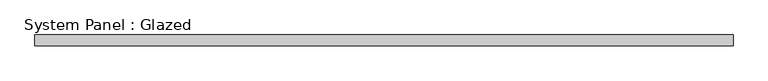
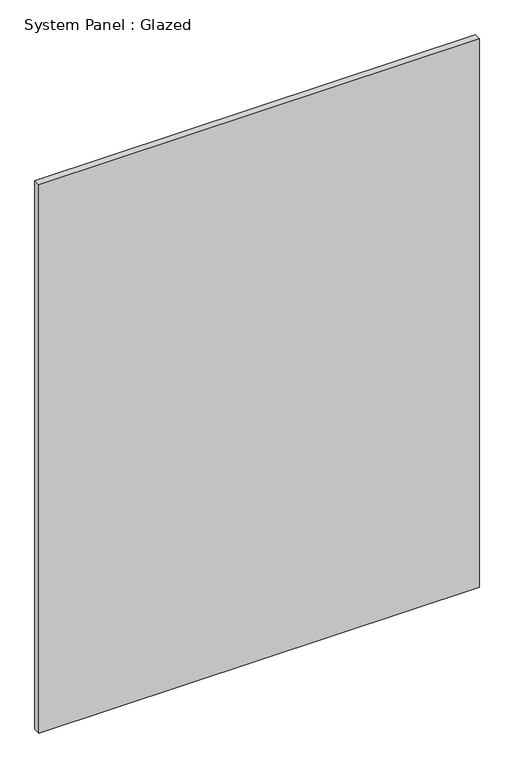
"""IFC4 building model written with IfcOpenShell, lengths in millimetres: plate geometry, System Panel : Glazed."""

from ifc_helpers import new_model, si_unit, origin, origin_with_axes, place, context, project, spatial, polyline, outline, extrude, source, transform, mapped, element, save


def system_panel_glazed_2d900ec6(model_context):
    return source(origin(), model_context, "Body", "SweptSolid", [
        extrude(outline(polyline([(807.775, -49.5), (-807.775, -49.5), (-807.775, -24.5), (807.775, -24.5), (807.775, -49.5)])), origin_with_axes(), (0.0, 0.0, 1.0), 2125.0),
    ])


if __name__ == "__main__":
    model = new_model("IFC4")
    model_context = context("Model", 3, world=origin())
    ifc_project = project(units=[si_unit("LENGTHUNIT", "METRE", prefix="MILLI")], contexts=[model_context])
    site = spatial("IfcSite", under=ifc_project)
    building = spatial("IfcBuilding", under=site)
    placement = place(None, origin())
    system_panel_glazed_shape = system_panel_glazed_2d900ec6(model_context)
    element("IfcPlate", 1, ObjectType="System Panel : Glazed", at=placement, inside=building, context=model_context, shape_type="MappedRepresentation", body=[
        mapped(system_panel_glazed_shape, transform((0.0, 0.0, 0.0), x_axis=(1.0, 0.0, 0.0), y_axis=(0.0, 1.0, 0.0), z_axis=(0.0, 0.0, 1.0))),
    ])
    save(model, "model.ifc")

# Revit data of these elements
# Type "System Panel : Glazed"
#   Keynote = "H11"
#   Construction Type Id = "GSP4R"
#   Analytic Construction = "1/8 in Pilkington single glazing"
#   Visual Light Transmittance = 0.9
#   Solar Heat Gain Coefficient = 0.86
#   Heat Transfer Coefficient (U) = 6.7069 W/(m²·K)
# Element 1 (IfcPlate, "System Panel : Glazed")
#   Materials on its faces: "Glass"
# Materials
#   "Glass": class "Glass", colour RGB 0 128 192, transparency 0.9, Description = "Soda Lime Glass", Cost = 0
